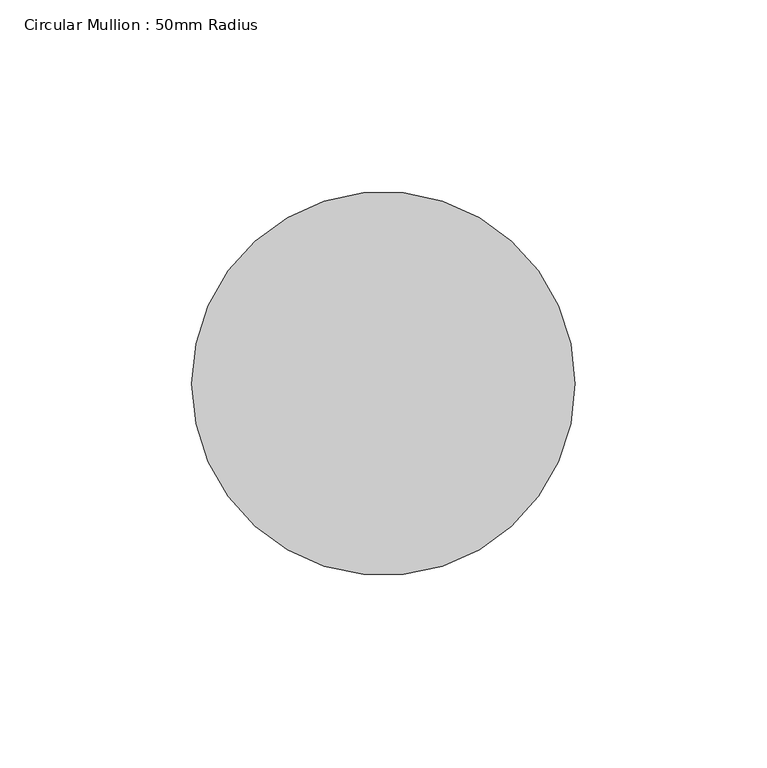
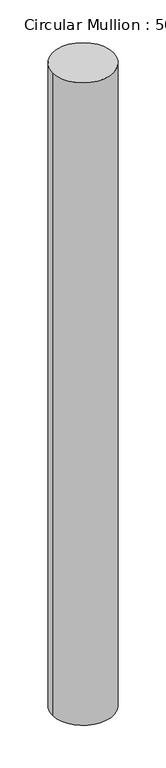
"""IFC4 building model written with IfcOpenShell, lengths in millimetres: member geometry, Circular Mullion : 50mm Radius."""

from ifc_helpers import new_model, si_unit, point, frame, origin, origin_2d, place, context, project, spatial, circle_curve, trimmed, segment, composite_curve, outline, extrude, source, transform, mapped, element, save


def circular_mullion_50mm_radius_ef1ca1fe(model_context):
    return source(origin(), model_context, "Body", "SweptSolid", [
        extrude(outline(composite_curve([segment(trimmed(circle_curve(origin_2d(), 50.0), [point((50.0, 0.0))], [point((-50.0, 0.0))], False, "CARTESIAN"), True, "CONTINUOUS"), segment(trimmed(circle_curve(origin_2d(), 50.0), [point((-50.0, 0.0))], [point((50.0, 0.0))], False, "CARTESIAN"), True, "CONTINUOUS")], self_intersect=False)), frame((0.0, 0.0, -1114.8900136), z_axis=(0.0, 0.0, 1.0), x_axis=(1.0, 0.0, 0.0)), (0.0, 0.0, 1.0), 1114.8900136),
    ])


if __name__ == "__main__":
    model = new_model("IFC4")
    model_context = context("Model", 3, world=origin())
    ifc_project = project(units=[si_unit("LENGTHUNIT", "METRE", prefix="MILLI")], contexts=[model_context])
    site = spatial("IfcSite", under=ifc_project)
    building = spatial("IfcBuilding", under=site)
    placement = place(None, origin())
    circular_mullion_50mm_radius_shape = circular_mullion_50mm_radius_ef1ca1fe(model_context)
    element("IfcMember", 1, ObjectType="Circular Mullion : 50mm Radius", at=placement, inside=building, context=model_context, shape_type="MappedRepresentation", body=[
        mapped(circular_mullion_50mm_radius_shape, transform((0.0, 0.0, 0.0), x_axis=(1.0, 0.0, 0.0), y_axis=(0.0, 1.0, 0.0), z_axis=(0.0, 0.0, 1.0))),
    ])
    save(model, "model.ifc")

# Revit data of these elements
# Type "Circular Mullion : 50mm Radius"
#   built-in parameter 1007350 = 0.164042 (stored number, unit not read)
# Element 1 (IfcMember, "Circular Mullion : 50mm Radius")
#   Materials on its faces: "Aluminium"
# Materials
#   "Aluminium": class "Metal", colour RGB 247 247 247, transparency 0, Description = "Aluminium 6061", Cost = 0
